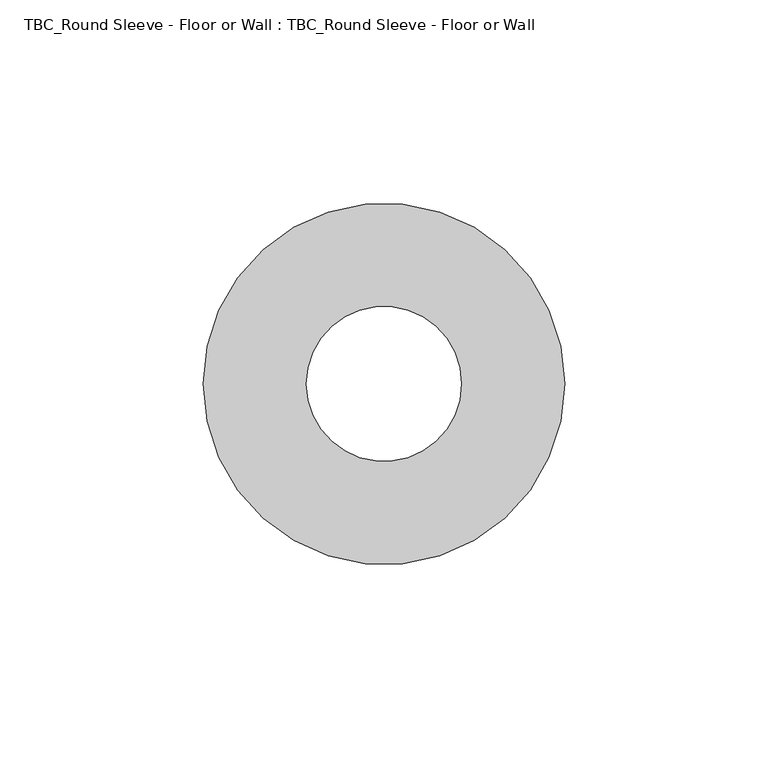
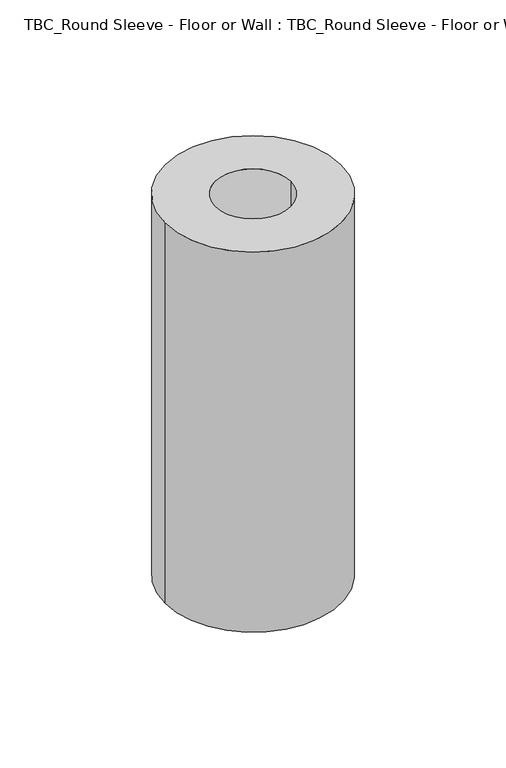
"""IFC4 building model written with IfcOpenShell, lengths in millimetres: proxy geometry, TBC_Round Sleeve - Floor or Wall : TBC_Round Sleeve - Floor or Wall."""

from ifc_helpers import new_model, si_unit, point, frame, origin, origin_2d, place, context, project, spatial, circle_curve, trimmed, segment, composite_curve, outline, extrude, source, transform, mapped, element, save


def tbc_round_sleeve_floor_or_wall_tbc_round_sleeve_floor_or_2e554980(model_context):
    return source(origin(), model_context, "Body", "SweptSolid", [
        extrude(outline(composite_curve([segment(trimmed(circle_curve(origin_2d(), 44.45), [point((-44.45, 0.0))], [point((44.45, 0.0))], False, "CARTESIAN"), True, "CONTINUOUS"), segment(trimmed(circle_curve(origin_2d(), 44.45), [point((44.45, 0.0))], [point((-44.45, 0.0))], False, "CARTESIAN"), True, "CONTINUOUS")], self_intersect=False), holes=[composite_curve([segment(trimmed(circle_curve(origin_2d(), 19.05), [point((-19.05, 0.0))], [point((19.05, 0.0))], True, "CARTESIAN"), True, "CONTINUOUS"), segment(trimmed(circle_curve(origin_2d(), 19.05), [point((19.05, 0.0))], [point((-19.05, 0.0))], True, "CARTESIAN"), True, "CONTINUOUS")], self_intersect=False)]), frame((0.0, 0.0, -203.2), z_axis=(0.0, 0.0, 1.0), x_axis=(1.0, 0.0, 0.0)), (0.0, 0.0, 1.0), 203.2),
    ])


if __name__ == "__main__":
    model = new_model("IFC4")
    model_context = context("Model", 3, world=origin())
    ifc_project = project(units=[si_unit("LENGTHUNIT", "METRE", prefix="MILLI")], contexts=[model_context])
    site = spatial("IfcSite", under=ifc_project)
    building = spatial("IfcBuilding", under=site)
    placement = place(None, origin())
    tbc_round_sleeve_floor_or_wall_tbc_round_sleeve_floor_or_shape = tbc_round_sleeve_floor_or_wall_tbc_round_sleeve_floor_or_2e554980(model_context)
    element("IfcBuildingElementProxy", 1, Name="TBC_Round Sleeve - Floor or Wall : TBC_Round Sleeve - Floor or Wall", ObjectType="TBC_Round Sleeve - Floor or Wall : TBC_Round Sleeve - Floor or Wall", at=placement, inside=building, context=model_context, shape_type="MappedRepresentation", body=[
        mapped(tbc_round_sleeve_floor_or_wall_tbc_round_sleeve_floor_or_shape, transform((0.0, 0.0, 0.0), x_axis=(1.0, 0.0, 0.0), y_axis=(0.0, 1.0, 0.0), z_axis=(0.0, 0.0, 1.0))),
    ])
    save(model, "model.ifc")

# Revit data of these elements
# Type "TBC_Round Sleeve - Floor or Wall : TBC_Round Sleeve - Floor or Wall"
#   Tag Dimension [instance default] = ""
#   MEP Type [instance default] = ""
#   MEP Element [instance default] = ""
#   MEP Category [instance default] = ""
#   Host Element Type [instance default] = ""
#   Host Element Id [instance default] = ""
#   Host Element Category [instance default] = ""
#   Control Line Y [instance default] = ""
#   Control Line X [instance default] = ""
#   Sleeve Radius [instance default] = 1' - 0"
#   Sleeve Edge [instance default] = 1' - 2"
#   Sleeve Depth [instance default] = 3' - 0"
#   Distance Y [instance default] = 0' - 0"
#   Distance X [instance default] = 0' - 0"
#   Default Elevation = 0
# Element 1 (IfcBuildingElementProxy, "TBC_Round Sleeve - Floor or Wall : TBC_Round Sleeve - Floor or Wall")
#   MEP Type = "Conduit"
#   MEP Element = "887104"
#   MEP Category = "Conduit"
#   Host Element Type = "8\" Plank"
#   Host Element Id = "721146"
#   Host Element Category = "Floors"
#   Sleeve Radius = 0' - 1 1/2"
#   Sleeve Edge = 0' - 3 1/2"
#   Sleeve Depth = 0' - 8"
